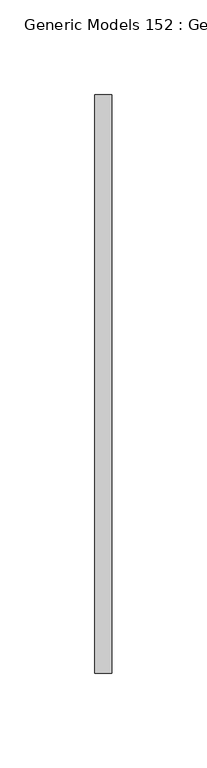
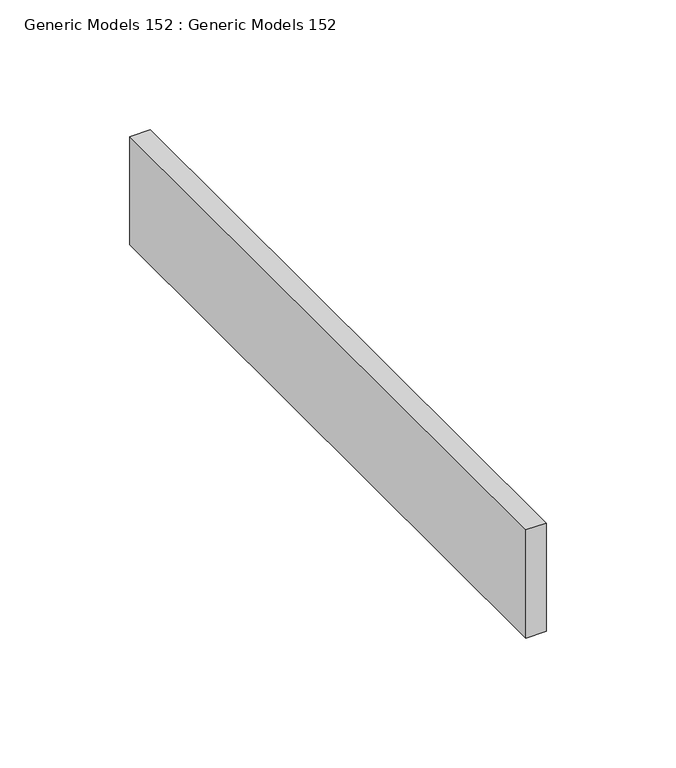
"""IFC4 building model written with IfcOpenShell, lengths in millimetres: proxy geometry, Generic Models 152 : Generic Models 152."""

from ifc_helpers import new_model, si_unit, frame, origin, place, context, project, spatial, polyline, outline, extrude, source, transform, mapped, element, save


def generic_models_152_generic_models_152_7f306fb8(model_context):
    return source(origin(), model_context, "Body", "SweptSolid", [
        extrude(outline(polyline([(4831.5063112, 704.5309662), (4840.4939304, 704.5309662), (4840.4939304, 399.7309662), (4831.5063112, 399.7309662), (4831.5063112, 704.5309662)])), frame((0.0, 0.0, 126205.996), z_axis=(0.0, 0.0, 1.0), x_axis=(1.0, 0.0, 0.0)), (0.0, 0.0, 1.0), 50.8),
    ])


if __name__ == "__main__":
    model = new_model("IFC4")
    model_context = context("Model", 3, world=origin())
    ifc_project = project(units=[si_unit("LENGTHUNIT", "METRE", prefix="MILLI")], contexts=[model_context])
    site = spatial("IfcSite", under=ifc_project)
    building = spatial("IfcBuilding", under=site)
    placement = place(None, origin())
    generic_models_152_generic_models_152_shape = generic_models_152_generic_models_152_7f306fb8(model_context)
    element("IfcBuildingElementProxy", 1, Name="Generic Models 152 : Generic Models 152", ObjectType="Generic Models 152 : Generic Models 152", at=placement, inside=building, context=model_context, shape_type="MappedRepresentation", body=[
        mapped(generic_models_152_generic_models_152_shape, transform((0.0, 0.0, 0.0), x_axis=(1.0, 0.0, 0.0), y_axis=(0.0, 1.0, 0.0), z_axis=(0.0, 0.0, 1.0))),
    ])
    save(model, "model.ifc")

# Revit data of these elements
# Element 1 (IfcBuildingElementProxy, "Generic Models 152 : Generic Models 152")
#   Materials on its faces: "_BLOCKING AS REQUIRED"
# Materials
#   "_BLOCKING AS REQUIRED": class "Generic", colour RGB 177 130 114, transparency 0, Cost = 0
